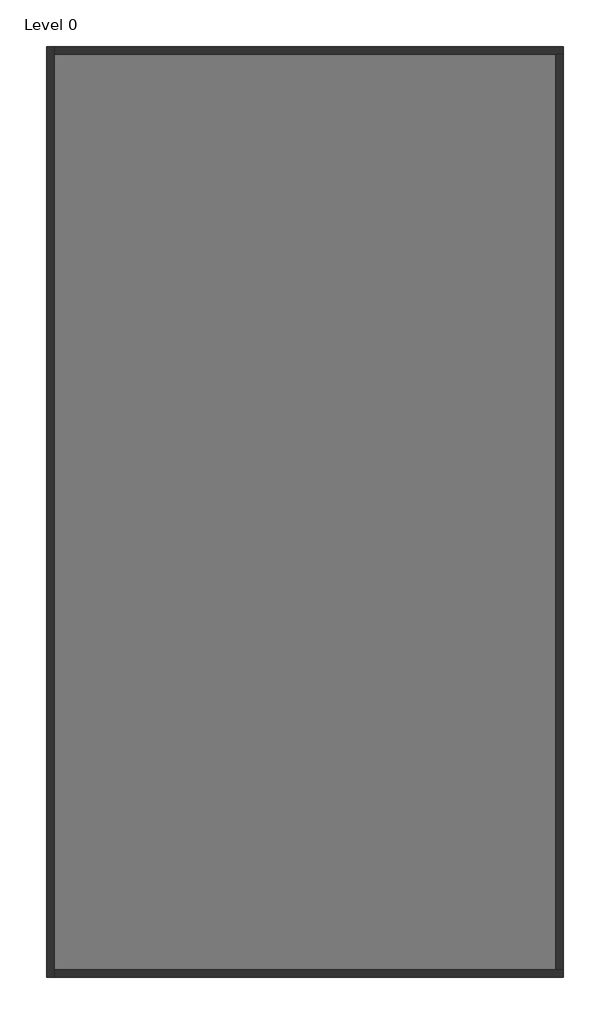
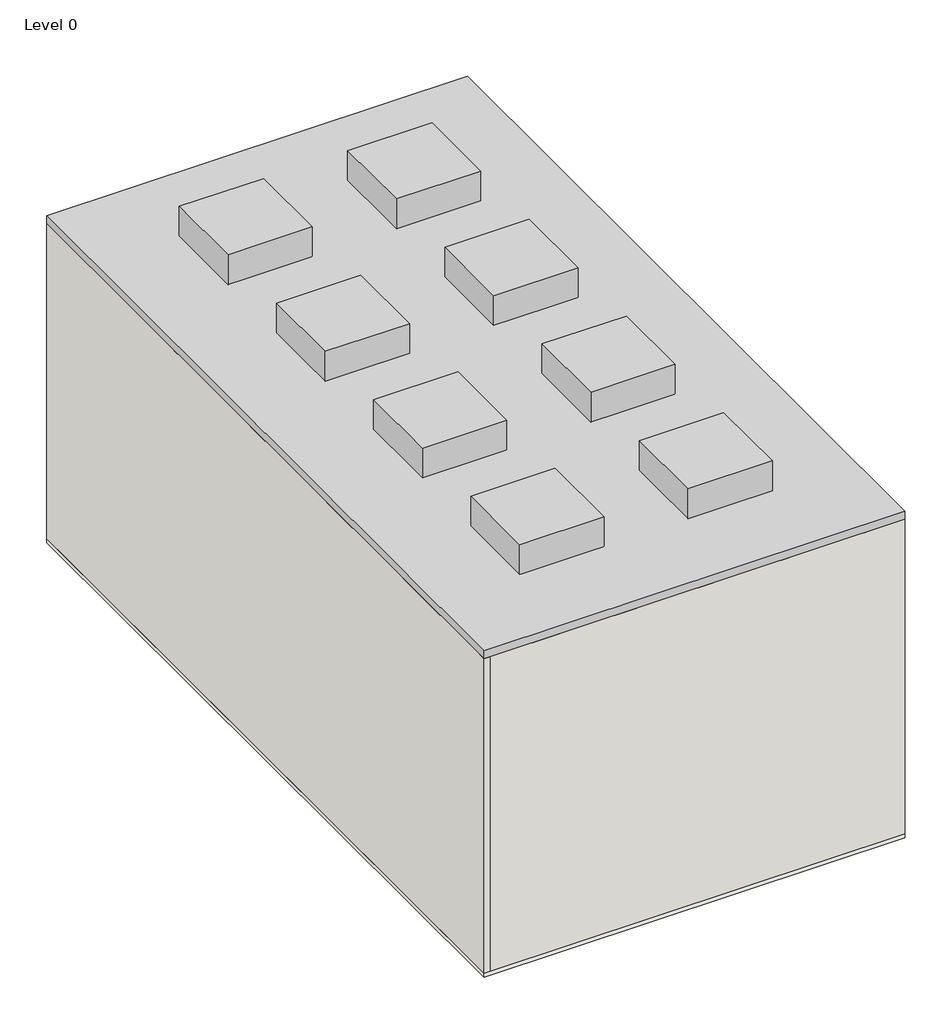
# One storey: 4 walls, 1 proxy, 1 slab.
"""IFC4 building model written with IfcOpenShell, lengths in millimetres."""

import ifcopenshell
import ifcopenshell.guid

model = None  # the IFC model being written
_history = None  # IfcOwnerHistory: only IFC2X3 demands one
_inside = {}  # id of a spatial element -> (the spatial element, [elements in it])
_under = {}  # id of a project, library or spatial element -> (it, [spatial elements below it])
_declared = {}  # id of a project -> (the project, [libraries it declares])
_typed = {}  # id of a type object -> (the type object, [elements of that type])
_made_of = {}  # id of a material, layer set ... -> (it, [elements and type objects made of it])


def new_model(schema):
    """Start an empty IFC model of exactly this schema.

    Asked for "IFC4X3", IfcOpenShell would pick the latest addendum, in which some entities
    have other attributes; the version numbers below select the first issue.
    IFC2X3 requires an IfcOwnerHistory on every rooted entity: one is made here for all.
    """
    global model, _history
    if schema == "IFC4X3":
        model = ifcopenshell.file(schema_version=(4, 3, 0, 0))
    else:
        model = ifcopenshell.file(schema=schema)
    _inside.clear()
    _under.clear()
    _declared.clear()
    _typed.clear()
    _made_of.clear()
    _history = None
    if model.schema == "IFC2X3":
        org = make("IfcOrganization", Name="unknown")
        user = make(
            "IfcPersonAndOrganization",
            ThePerson=make("IfcPerson", FamilyName="unknown"),
            TheOrganization=org,
        )
        app = make(
            "IfcApplication",
            ApplicationDeveloper=org,
            Version="unknown",
            ApplicationFullName="unknown",
            ApplicationIdentifier="unknown",
        )
        _history = make(
            "IfcOwnerHistory",
            OwningUser=user,
            OwningApplication=app,
            ChangeAction="ADDED",
            CreationDate=0,
        )
    return model


def make(cls, **values):
    """One entity of the class cls with the attributes given. An attribute that is None is left unset."""
    return model.create_entity(
        cls, **{name: value for name, value in values.items() if value is not None}
    )


def rooted(cls, **values):
    """An entity with a GlobalId (a new one), such as an element, a storey or a relation."""
    return make(cls, GlobalId=ifcopenshell.guid.new(), OwnerHistory=_history, **values)


def si_unit(unit_type, name, prefix=None):
    """IfcSIUnit, for example si_unit("LENGTHUNIT", "METRE", prefix="MILLI")."""
    return make("IfcSIUnit", UnitType=unit_type, Prefix=prefix, Name=name)


def assignment(units):
    """IfcUnitAssignment: the units of a project."""
    return None if units is None else make("IfcUnitAssignment", Units=units)


def point(xyz):
    """IfcCartesianPoint."""
    return None if xyz is None else make("IfcCartesianPoint", Coordinates=xyz)


def direction(xyz):
    """IfcDirection."""
    return None if xyz is None else make("IfcDirection", DirectionRatios=xyz)


def frame(location, z_axis=None, x_axis=None):
    """IfcAxis2Placement3D, a coordinate frame: its origin and axes. An axis left out is left unset."""
    return make(
        "IfcAxis2Placement3D",
        Location=point(location),
        Axis=direction(z_axis),
        RefDirection=direction(x_axis),
    )


def origin():
    """The frame at (0, 0, 0) with its axes left unset."""
    return frame((0.0, 0.0, 0.0))


def origin_with_axes():
    """The frame at (0, 0, 0) with the z axis (0, 0, 1) and the x axis (1, 0, 0) written out."""
    return frame((0.0, 0.0, 0.0), z_axis=(0.0, 0.0, 1.0), x_axis=(1.0, 0.0, 0.0))


def place(relative_to, where):
    """IfcLocalPlacement: puts the frame where relative to a parent placement (None: the world)."""
    return make(
        "IfcLocalPlacement", PlacementRelTo=relative_to, RelativePlacement=where
    )


def context(
    kind, dimensions, precision=None, world=None, true_north=None, identifier=None
):
    """IfcGeometricRepresentationContext, for example the 3D "Model" context."""
    return make(
        "IfcGeometricRepresentationContext",
        ContextIdentifier=identifier,
        ContextType=kind,
        CoordinateSpaceDimension=dimensions,
        Precision=precision,
        WorldCoordinateSystem=world,
        TrueNorth=true_north,
    )


def project(units=None, contexts=None):
    """IfcProject with its units and contexts."""
    return rooted(
        "IfcProject",
        Name="project",
        RepresentationContexts=contexts,
        UnitsInContext=assignment(units),
    )


def spatial(cls, under=None, at=None, **own):
    """A site, building, storey or space (cls), placed at a placement, below another one or the project."""
    s = rooted(cls, ObjectPlacement=at, **own)
    if under is not None:
        _under.setdefault(under.id(), (under, []))[1].append(s)
    return s


def polyline(points):
    """IfcPolyline through the points."""
    return make("IfcPolyline", Points=[point(p) for p in points])


def outline(outer, holes=None, kind="AREA"):
    """IfcArbitraryClosedProfileDef: a profile drawn as a closed curve; with holes, ...WithVoids."""
    if holes is None:
        return make("IfcArbitraryClosedProfileDef", ProfileType=kind, OuterCurve=outer)
    return make(
        "IfcArbitraryProfileDefWithVoids",
        ProfileType=kind,
        OuterCurve=outer,
        InnerCurves=holes,
    )


def extrude(swept, where, along, depth):
    """IfcExtrudedAreaSolid: the profile swept, set in the frame where, extruded along a direction by depth."""
    return make(
        "IfcExtrudedAreaSolid",
        SweptArea=swept,
        Position=where,
        ExtrudedDirection=direction(along),
        Depth=depth,
    )


def faces_of(points, faces, orient=None, outer=None):
    """IfcFace entities. A face is a list of loops; a loop is a list of indices into points, from 0.

    orient and outer hold one flag for each loop. By default every Orientation is true, the
    first loop of a face is its IfcFaceOuterBound and the others are IfcFaceBound.
    """
    made = []
    for i, loops in enumerate(faces):
        bounds = []
        for j, loop in enumerate(loops):
            is_outer = j == 0 if outer is None else outer[i][j]
            bounds.append(
                make(
                    "IfcFaceOuterBound" if is_outer else "IfcFaceBound",
                    Bound=make("IfcPolyLoop", Polygon=[points[k] for k in loop]),
                    Orientation=True if orient is None else orient[i][j],
                )
            )
        made.append(make("IfcFace", Bounds=bounds))
    return made


def faceted_brep(points, faces, orient=None, outer=None, voids=None):
    """IfcFacetedBrep: a solid bounded by flat faces; with voids (closed shells), ...WithVoids."""
    shared = [point(p) for p in points]
    hull = make("IfcClosedShell", CfsFaces=faces_of(shared, faces, orient, outer))
    if voids is None:
        return make("IfcFacetedBrep", Outer=hull)
    return make(
        "IfcFacetedBrepWithVoids",
        Outer=hull,
        Voids=[
            make(cls, CfsFaces=faces_of(shared, fs, o, b)) for cls, fs, o, b in voids
        ],
    )


def shape(context_of_items, identifier, shape_type, items):
    """IfcShapeRepresentation: the items that make up one representation, for example the "Body"."""
    return make(
        "IfcShapeRepresentation",
        ContextOfItems=context_of_items,
        RepresentationIdentifier=identifier,
        RepresentationType=shape_type,
        Items=items,
    )


def made_of(thing, what):
    """Note that an element or type object is made of a material, layer set ...; save() writes the relation."""
    if what is not None:
        _made_of.setdefault(what.id(), (what, []))[1].append(thing)
    return thing


def element(
    cls,
    number,
    at=None,
    inside=None,
    cuts=None,
    type_object=None,
    material=None,
    context=None,
    identifier="Body",
    shape_type=None,
    held_by="IfcProductDefinitionShape",
    body=None,
    shapes=None,
    **own,
):
    """One element of the class cls, such as IfcWall. Its Tag is "e" and its number.

    at: its placement. inside: the storey or other place that contains it. cuts: it is an
    opening in that element (IfcRelVoidsElement). A single representation is given by context,
    identifier, shape_type and body (its items); several are given by shapes. held_by: the class
    of the entity that holds the representations. save() writes the other relations.
    """
    e = rooted(cls, Tag="e%d" % number, ObjectPlacement=at, **own)
    if body is not None:
        shapes = [shape(context, identifier, shape_type, body)]
    if shapes is not None:
        e.Representation = make(held_by, Representations=shapes)
    if inside is not None:
        _inside.setdefault(inside.id(), (inside, []))[1].append(e)
    if cuts is not None:
        rooted(
            "IfcRelVoidsElement", RelatingBuildingElement=cuts, RelatedOpeningElement=e
        )
    if type_object is not None:
        _typed.setdefault(type_object.id(), (type_object, []))[1].append(e)
    return made_of(e, material)


def aggregate(whole, parts):
    """IfcRelAggregates: a whole, such as a stair, and the parts it consists of."""
    return rooted("IfcRelAggregates", RelatingObject=whole, RelatedObjects=parts)


def save(model, path):
    """Write the relations noted so far, then the file.

    IfcRelAggregates (storeys below a building ...), IfcRelContainedInSpatialStructure (elements
    in a storey), IfcRelDefinesByType, IfcRelAssociatesMaterial and IfcRelDeclares: one each for
    every whole, place, type object, material and project.
    """
    for whole, parts in _under.values():
        aggregate(whole, parts)
    for where, things in _inside.values():
        rooted(
            "IfcRelContainedInSpatialStructure",
            RelatedElements=things,
            RelatingStructure=where,
        )
    for kind, things in _typed.values():
        rooted("IfcRelDefinesByType", RelatedObjects=things, RelatingType=kind)
    for what, things in _made_of.values():
        rooted("IfcRelAssociatesMaterial", RelatedObjects=things, RelatingMaterial=what)
    for by, libraries in _declared.values():
        rooted("IfcRelDeclares", RelatingContext=by, RelatedDefinitions=libraries)
    model.write(path)


model = new_model("IFC4")

# Units and contexts
model_context = context("Model", 3, world=origin())
ifc_project = project(units=[si_unit("LENGTHUNIT", "METRE", prefix="MILLI")], contexts=[model_context])

# Site, building, storey
site = spatial("IfcSite", under=ifc_project)
building = spatial("IfcBuilding", under=site)
storey = spatial("IfcBuildingStorey", under=building, Name="Level 0", Elevation=100.0)

# Proxy
placement = place(None, origin())
element("IfcBuildingElementProxy", 1, Name="LowUrbanDensityBuilding : LowUrbanDensityBuilding", ObjectType="LowUrbanDensityBuilding : LowUrbanDensityBuilding", at=placement, inside=storey, context=model_context, shape_type="SweptSolid", body=[
    extrude(outline(polyline([(7325.2659446, 3676.2074539), (7325.2659446, -14323.7925461), (-2674.7340554, -14323.7925461), (-2674.7340554, 3676.2074539), (7325.2659446, 3676.2074539)])), origin_with_axes(), (0.0, 0.0, 1.0), 8200.0),
    extrude(outline(polyline([(1325.2659446, 1676.2074539), (1325.2659446, -323.7925461), (-674.7340554, -323.7925461), (-674.7340554, 1676.2074539), (1325.2659446, 1676.2074539)])), frame((0.0, 0.0, 8200.0), z_axis=(0.0, 0.0, 1.0), x_axis=(1.0, 0.0, 0.0)), (0.0, 0.0, 1.0), 749.8),
    extrude(outline(polyline([(5325.2659446, 1676.2074539), (5325.2659446, -323.7925461), (3325.2659446, -323.7925461), (3325.2659446, 1676.2074539), (5325.2659446, 1676.2074539)])), frame((0.0, 0.0, 8200.0), z_axis=(0.0, 0.0, 1.0), x_axis=(1.0, 0.0, 0.0)), (0.0, 0.0, 1.0), 749.8),
    extrude(outline(polyline([(1325.2659446, -2323.7925461), (1325.2659446, -4323.7925461), (-674.7340554, -4323.7925461), (-674.7340554, -2323.7925461), (1325.2659446, -2323.7925461)])), frame((0.0, 0.0, 8200.0), z_axis=(0.0, 0.0, 1.0), x_axis=(1.0, 0.0, 0.0)), (0.0, 0.0, 1.0), 749.8),
    extrude(outline(polyline([(5325.2659446, -2323.7925461), (5325.2659446, -4323.7925461), (3325.2659446, -4323.7925461), (3325.2659446, -2323.7925461), (5325.2659446, -2323.7925461)])), frame((0.0, 0.0, 8200.0), z_axis=(0.0, 0.0, 1.0), x_axis=(1.0, 0.0, 0.0)), (0.0, 0.0, 1.0), 749.8),
    extrude(outline(polyline([(1325.2659446, -6323.7925461), (1325.2659446, -8323.7925461), (-674.7340554, -8323.7925461), (-674.7340554, -6323.7925461), (1325.2659446, -6323.7925461)])), frame((0.0, 0.0, 8200.0), z_axis=(0.0, 0.0, 1.0), x_axis=(1.0, 0.0, 0.0)), (0.0, 0.0, 1.0), 749.8),
    extrude(outline(polyline([(5325.2659446, -6323.7925461), (5325.2659446, -8323.7925461), (3325.2659446, -8323.7925461), (3325.2659446, -6323.7925461), (5325.2659446, -6323.7925461)])), frame((0.0, 0.0, 8200.0), z_axis=(0.0, 0.0, 1.0), x_axis=(1.0, 0.0, 0.0)), (0.0, 0.0, 1.0), 749.8),
    extrude(outline(polyline([(1325.2659446, -10323.7925461), (1325.2659446, -12323.7925461), (-674.7340554, -12323.7925461), (-674.7340554, -10323.7925461), (1325.2659446, -10323.7925461)])), frame((0.0, 0.0, 8200.0), z_axis=(0.0, 0.0, 1.0), x_axis=(1.0, 0.0, 0.0)), (0.0, 0.0, 1.0), 749.8),
    extrude(outline(polyline([(5325.2659446, -10323.7925461), (5325.2659446, -12323.7925461), (3325.2659446, -12323.7925461), (3325.2659446, -10323.7925461), (5325.2659446, -10323.7925461)])), frame((0.0, 0.0, 8200.0), z_axis=(0.0, 0.0, 1.0), x_axis=(1.0, 0.0, 0.0)), (0.0, 0.0, 1.0), 749.8),
])

# Slab
element("IfcSlab", 2, ObjectType="Floor-Concrete_100Con", at=placement, inside=storey, context=model_context, shape_type="SweptSolid", body=[
    extrude(outline(polyline([(7325.2659446, 3676.2074539), (7325.2659446, -14323.7925461), (-2674.7340554, -14323.7925461), (-2674.7340554, 3676.2074539), (7325.2659446, 3676.2074539)])), origin_with_axes(), (0.0, 0.0, 1.0), 100.0),
])

# Walls
element("IfcWall", 3, ObjectType="Wall-Ext_25Rdr-100Blk-19P", at=placement, inside=storey, context=model_context, shape_type="Brep", body=[
    faceted_brep([(-2674.7340554, 3676.2074539, 100.0), (-2674.7340554, -14323.7925461, 100.0), (-2674.7340554, -14323.7925461, 8000.0), (-2674.7340554, 3676.2074539, 8000.0), (-2530.4340554, 3676.2074539, 100.0), (-2530.4340554, 3676.2074539, 8000.0), (-2530.4340554, 3531.9074539, 8000.0), (-2530.4340554, -14179.4925461, 8000.0), (-2530.4340554, -14323.7925461, 8000.0), (-2530.4340554, -14323.7925461, 100.0), (-2530.4340554, -14179.4925461, 100.0), (-2530.4340554, 3531.9074539, 100.0)], [[[0, 1, 2, 3]], [[4, 5, 6, 7, 8, 9, 10, 11]], [[1, 0, 4, 11, 10, 9]], [[3, 2, 8, 7, 6, 5]], [[2, 1, 9, 8]], [[0, 3, 5, 4]]]),
])
element("IfcWall", 4, ObjectType="Wall-Ext_25Rdr-100Blk-19P", at=placement, inside=storey, context=model_context, shape_type="Brep", body=[
    faceted_brep([(-2530.4340554, -14323.7925461, 100.0), (7325.2659446, -14323.7925461, 100.0), (7325.2659446, -14323.7925461, 8000.0), (-2530.4340554, -14323.7925461, 8000.0), (-2530.4340554, -14179.4925461, 100.0), (-2530.4340554, -14179.4925461, 8000.0), (7180.9659446, -14179.4925461, 8000.0), (7325.2659446, -14179.4925461, 8000.0), (7325.2659446, -14179.4925461, 100.0), (7180.9659446, -14179.4925461, 100.0)], [[[0, 1, 2, 3]], [[4, 5, 6, 7, 8, 9]], [[1, 0, 4, 9, 8]], [[3, 2, 7, 6, 5]], [[0, 3, 5, 4]], [[2, 1, 8, 7]]]),
])
element("IfcWall", 5, ObjectType="Wall-Ext_25Rdr-100Blk-19P", at=placement, inside=storey, context=model_context, shape_type="Brep", body=[
    faceted_brep([(7325.2659446, 3676.2074539, 100.0), (-2530.4340554, 3676.2074539, 100.0), (-2530.4340554, 3676.2074539, 8000.0), (7325.2659446, 3676.2074539, 8000.0), (7325.2659446, 3531.9074539, 100.0), (7325.2659446, 3531.9074539, 8000.0), (7180.9659446, 3531.9074539, 8000.0), (-2530.4340554, 3531.9074539, 8000.0), (-2530.4340554, 3531.9074539, 100.0), (7180.9659446, 3531.9074539, 100.0)], [[[0, 1, 2, 3]], [[4, 5, 6, 7, 8, 9]], [[1, 0, 4, 9, 8]], [[3, 2, 7, 6, 5]], [[2, 1, 8, 7]], [[0, 3, 5, 4]]]),
])
element("IfcWall", 6, ObjectType="Wall-Ext_25Rdr-100Blk-19P", at=placement, inside=storey, context=model_context, shape_type="SweptSolid", body=[
    extrude(outline(polyline([(7325.2659446, 3531.9074539), (7325.2659446, -14179.4925461), (7180.9659446, -14179.4925461), (7180.9659446, 3531.9074539), (7325.2659446, 3531.9074539)])), frame((0.0, 0.0, 100.0), z_axis=(0.0, 0.0, 1.0), x_axis=(1.0, 0.0, 0.0)), (0.0, 0.0, 1.0), 7900.0),
])

save(model, "model.ifc")

# Revit data of these elements
# Project information
#   Project Issue Date = "Issue Date"
#   Project Status = "Project Status"
#   Client Name = "Owner"
#   Project Address = "Enter address here"
#   Project Name = "Project Name"
#   Project Number = "Project Number"
# Type "Floor-Concrete_100Con"
#   Keynote = "E60/130"
#   Function = 0
#   Layers, outside or top first: 100 mm "Concrete" (function 1)
# Type "Wall-Ext_25Rdr-100Blk-19P"
#   Keynote = "F10"
#   Layers, outside or top first: 25.3 mm "Render, Beige, Smooth" (function 5); 100 mm "Concrete Masonry Units _Low Density" (function 1); 19 mm "Plaster" (function 5)
# Element 1 (IfcBuildingElementProxy, "LowUrbanDensityBuilding : LowUrbanDensityBuilding")
#   Phase Created = New Construction
#   Materials on its faces: "Default Form"
# Element 2 (IfcSlab, "Floor-Concrete_100Con")
#   Height Offset From Level = 0 mm
#   Phase Created = New Construction
#   Materials on its faces: "Concrete"
# Element 3 (IfcWall, "Wall-Ext_25Rdr-100Blk-19P")
#   Top Offset = 0 mm
#   Base Offset = 0 mm
#   wall height = 7900 mm
#   Phase Created = New Construction
#   Base Constraint = Level 0
#   Top Constraint = Level 2
#   Materials on its faces: "Render, Beige, Smooth", "Default Wall", "Plaster"
# Elements 4, 5, 6 (IfcWall, "Wall-Ext_25Rdr-100Blk-19P")
#   Top Offset = 0 mm
#   Base Offset = 0 mm
#   wall height = 7900 mm
#   Phase Created = New Construction
#   Base Constraint = Level 0
#   Top Constraint = Level 2
#   Materials on its faces: "Default Wall", "Render, Beige, Smooth", "Plaster"
# Materials
#   "Concrete": class "Concrete", colour RGB 120 120 120, transparency 0, Description = "Portland Cement Concrete", Cost = 0
#   "Render, Beige, Smooth": class "Generic", colour RGB 213 198 180, transparency 0, Description = "physical material", Cost = 0
#   "Concrete Masonry Units _Low Density": class "Masonry", colour RGB 181 181 181, transparency 0, Description = "Concrete masonry units", Cost = 0
#   "Plaster": class "Generic", colour RGB 249 249 249, transparency 0, Description = "Plaster", Cost = 0
#   "Default Form": class "Generic", colour RGB 185 189 196, transparency 0.5, Cost = 0
#   "Default Wall": class "Miscellaneous", colour RGB 128 128 128, transparency 0, Comments = "Rendering appearance not upgraded Rendering appearance not upgraded ", Cost = 0
